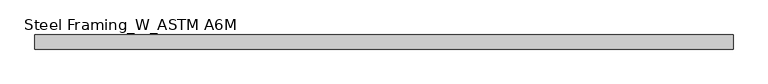
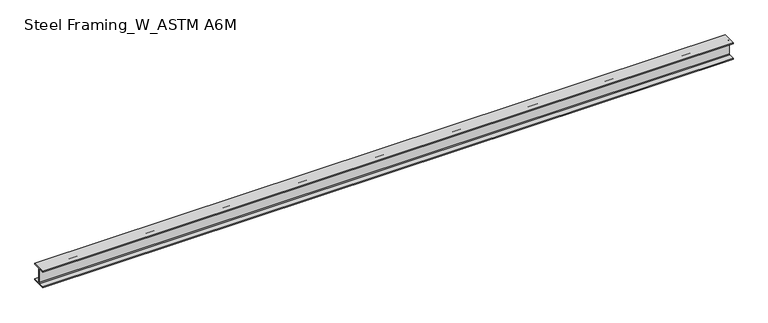
"""IFC4 building model written with IfcOpenShell, lengths in millimetres: beam geometry, Steel Framing_W_ASTM A6M : H_SB_AR_S02_W250x49.1_RB3."""

from ifc_helpers import new_model, si_unit, point, frame, frame_2d, origin, place, context, project, spatial, polyline, circle_curve, trimmed, segment, composite_curve, outline, extrude, source, transform, mapped, element, save


def steel_framing_w_astm_a6m_504daf18(model_context):
    return source(origin(), model_context, "Body", "SweptSolid", [
        extrude(outline(composite_curve([segment(polyline([(101.0, -112.5), (101.0, -123.5), (-101.0, -123.5), (-101.0, -112.5), (-16.385, -112.5)]), True, "CONTINUOUS"), segment(trimmed(circle_curve(frame_2d((-16.385, -99.8)), 12.7), [point((-16.385, -112.5))], [point((-3.685, -99.8))], True, "CARTESIAN"), True, "CONTINUOUS"), segment(polyline([(-3.685, -99.8), (-3.685, 99.8)]), True, "CONTINUOUS"), segment(trimmed(circle_curve(frame_2d((-16.385, 99.8)), 12.7), [point((-3.685, 99.8))], [point((-16.385, 112.5))], True, "CARTESIAN"), True, "CONTINUOUS"), segment(polyline([(-16.385, 112.5), (-101.0, 112.5), (-101.0, 123.5), (101.0, 123.5), (101.0, 112.5), (16.385, 112.5)]), True, "CONTINUOUS"), segment(trimmed(circle_curve(frame_2d((16.385, 99.8)), 12.7), [point((16.385, 112.5))], [point((3.685, 99.8))], True, "CARTESIAN"), True, "CONTINUOUS"), segment(polyline([(3.685, 99.8), (3.685, -99.8)]), True, "CONTINUOUS"), segment(trimmed(circle_curve(frame_2d((16.385, -99.8)), 12.7), [point((3.685, -99.8))], [point((16.385, -112.5))], True, "CARTESIAN"), True, "CONTINUOUS"), segment(polyline([(16.385, -112.5), (101.0, -112.5)]), True, "CONTINUOUS")], self_intersect=False)), frame((-5000.0, 0.0, 0.0), z_axis=(1.0, 0.0, 0.0), x_axis=(0.0, 1.0, 0.0)), (0.0, 0.0, 1.0), 9987.2),
    ])


if __name__ == "__main__":
    model = new_model("IFC4")
    model_context = context("Model", 3, world=origin())
    ifc_project = project(units=[si_unit("LENGTHUNIT", "METRE", prefix="MILLI")], contexts=[model_context])
    site = spatial("IfcSite", under=ifc_project)
    building = spatial("IfcBuilding", under=site)
    placement = place(None, origin())
    steel_framing_w_astm_a6m_shape = steel_framing_w_astm_a6m_504daf18(model_context)
    element("IfcBeam", 1, ObjectType="Steel Framing_W_ASTM A6M : H_SB_AR_S02_W250x49.1_RB3", at=placement, inside=building, context=model_context, shape_type="MappedRepresentation", body=[
        mapped(steel_framing_w_astm_a6m_shape, transform((0.0, 0.0, 0.0), x_axis=(1.0, 0.0, 0.0), y_axis=(0.0, 1.0, 0.0), z_axis=(0.0, 0.0, 1.0))),
    ])
    save(model, "model.ifc")

# Revit data of these elements
# Type "Steel Framing_W_ASTM A6M : H_SB_AR_S02_W250x49.1_RB3"
#   Type Mark = "RB3"
#   Section Name Key = "W10x33"
#   Width = 20.2 cm
#   Web Thickness = 0.737 cm
#   Web Fillet = 1.27 cm
#   Warping Constant = 212000.0 cm⁶
#   Torsional Moment of Inertia = 24.30 cm⁴
#   Section Area = 62.6 cm²
#   Plastic Modulus weak axis = 229.0 cm³
#   Plastic Modulus strong axis = 636.0 cm³
#   Perimeter = 1.27 m²/m
#   Nominal Weight = 49.10 kgf/m
#   Moment of Inertia weak axis = 1520.00 cm⁴
#   Moment of Inertia strong axis = 7120.00 cm⁴
#   Height = 24.7 cm
#   Flange Thickness = 1.1 cm
#   Elastic Modulus weak axis = 151.0 cm³
#   Elastic Modulus strong axis = 574.0 cm³
#   Centroid Vertical = 12.35 cm
#   Centroid Horizontal = 10.1 cm
#   Length [instance default] = 1500 mm
#   Structural Material [instance default] = Steel, 45-345
#   Bolt Spacing = 0
#   Assembly Code = ""
# Element 1 (IfcBeam, "Steel Framing_W_ASTM A6M : H_SB_AR_S02_W250x49.1_RB3")
#   Materials on its faces: "Steel, 45-345"
# Materials
#   "Steel, 45-345": class "Metal", colour RGB 189 187 185, transparency 0, Description = "Steel 345 MPa", Cost = 0
